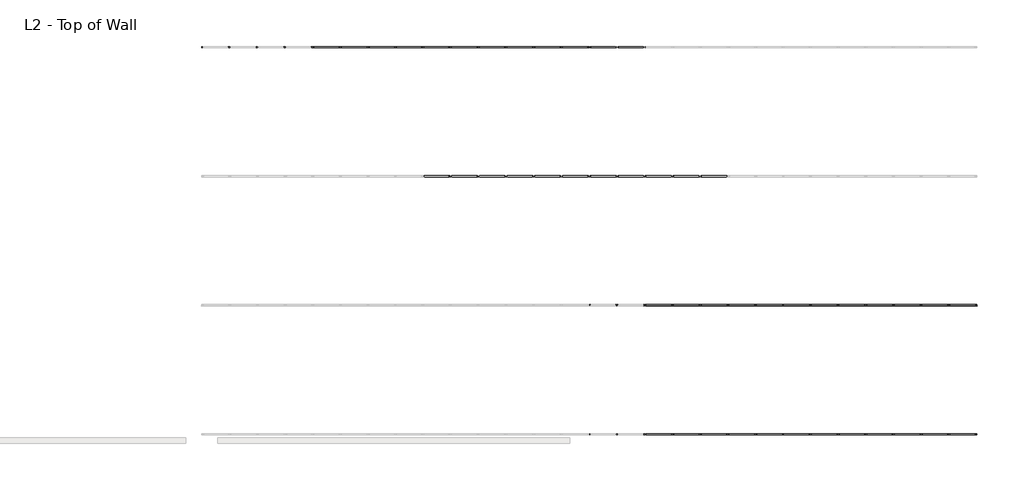
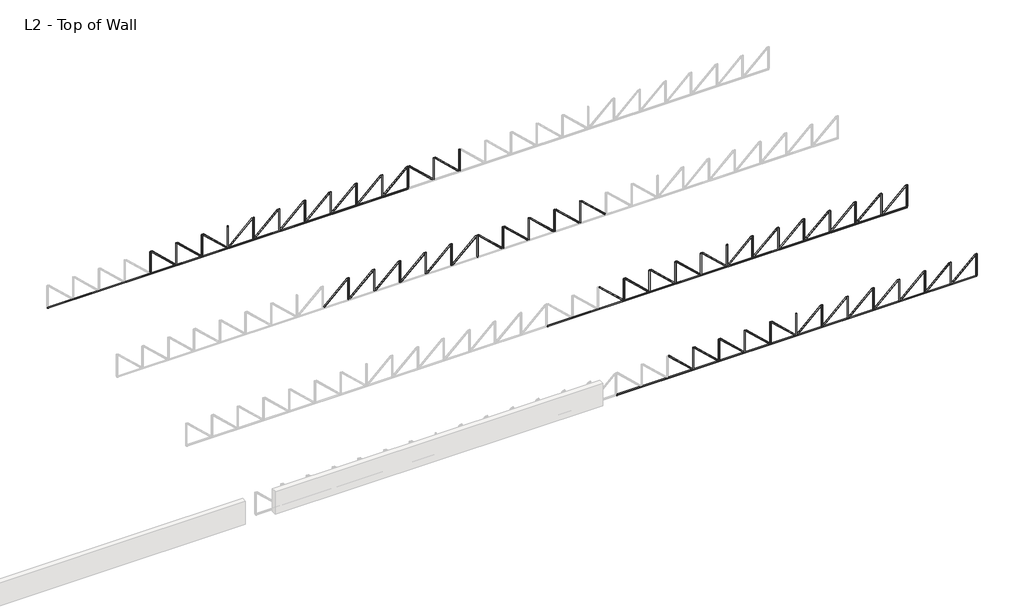
# One storey, part 2 of 4: 99 beams.
"""IFC4 building model written with IfcOpenShell, lengths in millimetres."""

import ifcopenshell
import ifcopenshell.guid

model = None  # the IFC model being written
_history = None  # IfcOwnerHistory: only IFC2X3 demands one
_inside = {}  # id of a spatial element -> (the spatial element, [elements in it])
_under = {}  # id of a project, library or spatial element -> (it, [spatial elements below it])
_declared = {}  # id of a project -> (the project, [libraries it declares])
_typed = {}  # id of a type object -> (the type object, [elements of that type])
_made_of = {}  # id of a material, layer set ... -> (it, [elements and type objects made of it])


def new_model(schema):
    """Start an empty IFC model of exactly this schema.

    Asked for "IFC4X3", IfcOpenShell would pick the latest addendum, in which some entities
    have other attributes; the version numbers below select the first issue.
    IFC2X3 requires an IfcOwnerHistory on every rooted entity: one is made here for all.
    """
    global model, _history
    if schema == "IFC4X3":
        model = ifcopenshell.file(schema_version=(4, 3, 0, 0))
    else:
        model = ifcopenshell.file(schema=schema)
    _inside.clear()
    _under.clear()
    _declared.clear()
    _typed.clear()
    _made_of.clear()
    _history = None
    if model.schema == "IFC2X3":
        org = make("IfcOrganization", Name="unknown")
        user = make(
            "IfcPersonAndOrganization",
            ThePerson=make("IfcPerson", FamilyName="unknown"),
            TheOrganization=org,
        )
        app = make(
            "IfcApplication",
            ApplicationDeveloper=org,
            Version="unknown",
            ApplicationFullName="unknown",
            ApplicationIdentifier="unknown",
        )
        _history = make(
            "IfcOwnerHistory",
            OwningUser=user,
            OwningApplication=app,
            ChangeAction="ADDED",
            CreationDate=0,
        )
    return model


def make(cls, **values):
    """One entity of the class cls with the attributes given. An attribute that is None is left unset."""
    return model.create_entity(
        cls, **{name: value for name, value in values.items() if value is not None}
    )


def rooted(cls, **values):
    """An entity with a GlobalId (a new one), such as an element, a storey or a relation."""
    return make(cls, GlobalId=ifcopenshell.guid.new(), OwnerHistory=_history, **values)


def si_unit(unit_type, name, prefix=None):
    """IfcSIUnit, for example si_unit("LENGTHUNIT", "METRE", prefix="MILLI")."""
    return make("IfcSIUnit", UnitType=unit_type, Prefix=prefix, Name=name)


def assignment(units):
    """IfcUnitAssignment: the units of a project."""
    return None if units is None else make("IfcUnitAssignment", Units=units)


def point(xyz):
    """IfcCartesianPoint."""
    return None if xyz is None else make("IfcCartesianPoint", Coordinates=xyz)


def direction(xyz):
    """IfcDirection."""
    return None if xyz is None else make("IfcDirection", DirectionRatios=xyz)


def frame(location, z_axis=None, x_axis=None):
    """IfcAxis2Placement3D, a coordinate frame: its origin and axes. An axis left out is left unset."""
    return make(
        "IfcAxis2Placement3D",
        Location=point(location),
        Axis=direction(z_axis),
        RefDirection=direction(x_axis),
    )


def frame_2d(location, x_axis=None):
    """IfcAxis2Placement2D, a coordinate frame in the plane: its origin and x axis."""
    return make(
        "IfcAxis2Placement2D", Location=point(location), RefDirection=direction(x_axis)
    )


def origin():
    """The frame at (0, 0, 0) with its axes left unset."""
    return frame((0.0, 0.0, 0.0))


def origin_2d():
    """The frame at (0, 0) in the plane with its x axis left unset."""
    return frame_2d((0.0, 0.0))


def place(relative_to, where):
    """IfcLocalPlacement: puts the frame where relative to a parent placement (None: the world)."""
    return make(
        "IfcLocalPlacement", PlacementRelTo=relative_to, RelativePlacement=where
    )


def context(
    kind, dimensions, precision=None, world=None, true_north=None, identifier=None
):
    """IfcGeometricRepresentationContext, for example the 3D "Model" context."""
    return make(
        "IfcGeometricRepresentationContext",
        ContextIdentifier=identifier,
        ContextType=kind,
        CoordinateSpaceDimension=dimensions,
        Precision=precision,
        WorldCoordinateSystem=world,
        TrueNorth=true_north,
    )


def project(units=None, contexts=None):
    """IfcProject with its units and contexts."""
    return rooted(
        "IfcProject",
        Name="project",
        RepresentationContexts=contexts,
        UnitsInContext=assignment(units),
    )


def spatial(cls, under=None, at=None, **own):
    """A site, building, storey or space (cls), placed at a placement, below another one or the project."""
    s = rooted(cls, ObjectPlacement=at, **own)
    if under is not None:
        _under.setdefault(under.id(), (under, []))[1].append(s)
    return s


def circle_curve(where, radius):
    """IfcCircle in the frame where."""
    return make("IfcCircle", Position=where, Radius=radius)


def trimmed(basis, trim1, trim2, sense, master):
    """IfcTrimmedCurve: the piece of a basis curve between two trims."""
    return make(
        "IfcTrimmedCurve",
        BasisCurve=basis,
        Trim1=trim1,
        Trim2=trim2,
        SenseAgreement=sense,
        MasterRepresentation=master,
    )


def segment(curve, same_sense, transition):
    """IfcCompositeCurveSegment."""
    return make(
        "IfcCompositeCurveSegment",
        Transition=transition,
        SameSense=same_sense,
        ParentCurve=curve,
    )


def composite_curve(segments, self_intersect=None):
    """IfcCompositeCurve: segments joined end to end."""
    return make("IfcCompositeCurve", Segments=segments, SelfIntersect=self_intersect)


def outline(outer, holes=None, kind="AREA"):
    """IfcArbitraryClosedProfileDef: a profile drawn as a closed curve; with holes, ...WithVoids."""
    if holes is None:
        return make("IfcArbitraryClosedProfileDef", ProfileType=kind, OuterCurve=outer)
    return make(
        "IfcArbitraryProfileDefWithVoids",
        ProfileType=kind,
        OuterCurve=outer,
        InnerCurves=holes,
    )


def extrude(swept, where, along, depth):
    """IfcExtrudedAreaSolid: the profile swept, set in the frame where, extruded along a direction by depth."""
    return make(
        "IfcExtrudedAreaSolid",
        SweptArea=swept,
        Position=where,
        ExtrudedDirection=direction(along),
        Depth=depth,
    )


def shape(context_of_items, identifier, shape_type, items):
    """IfcShapeRepresentation: the items that make up one representation, for example the "Body"."""
    return make(
        "IfcShapeRepresentation",
        ContextOfItems=context_of_items,
        RepresentationIdentifier=identifier,
        RepresentationType=shape_type,
        Items=items,
    )


def source(mapping_origin, context_of_items, identifier, shape_type, items):
    """IfcRepresentationMap: a shape defined once, which mapped items show again and again."""
    return make(
        "IfcRepresentationMap",
        MappingOrigin=mapping_origin,
        MappedRepresentation=shape(context_of_items, identifier, shape_type, items),
    )


def transform(
    local_origin,
    x_axis=None,
    y_axis=None,
    z_axis=None,
    scale=None,
    scale2=None,
    scale3=None,
    uniform=True,
):
    """IfcCartesianTransformationOperator3D, or its non-uniform kind. x_axis, y_axis, z_axis: its Axis1, 2, 3."""
    if uniform:
        return make(
            "IfcCartesianTransformationOperator3D",
            Axis1=direction(x_axis),
            Axis2=direction(y_axis),
            LocalOrigin=point(local_origin),
            Scale=scale,
            Axis3=direction(z_axis),
        )
    return make(
        "IfcCartesianTransformationOperator3DnonUniform",
        Axis1=direction(x_axis),
        Axis2=direction(y_axis),
        LocalOrigin=point(local_origin),
        Scale=scale,
        Axis3=direction(z_axis),
        Scale2=scale2,
        Scale3=scale3,
    )


def mapped(mapping_source, mapping_target):
    """IfcMappedItem: shows the shape of a source again, moved by a transform."""
    return make(
        "IfcMappedItem", MappingSource=mapping_source, MappingTarget=mapping_target
    )


def made_of(thing, what):
    """Note that an element or type object is made of a material, layer set ...; save() writes the relation."""
    if what is not None:
        _made_of.setdefault(what.id(), (what, []))[1].append(thing)
    return thing


def element(
    cls,
    number,
    at=None,
    inside=None,
    cuts=None,
    type_object=None,
    material=None,
    context=None,
    identifier="Body",
    shape_type=None,
    held_by="IfcProductDefinitionShape",
    body=None,
    shapes=None,
    **own,
):
    """One element of the class cls, such as IfcWall. Its Tag is "e" and its number.

    at: its placement. inside: the storey or other place that contains it. cuts: it is an
    opening in that element (IfcRelVoidsElement). A single representation is given by context,
    identifier, shape_type and body (its items); several are given by shapes. held_by: the class
    of the entity that holds the representations. save() writes the other relations.
    """
    e = rooted(cls, Tag="e%d" % number, ObjectPlacement=at, **own)
    if body is not None:
        shapes = [shape(context, identifier, shape_type, body)]
    if shapes is not None:
        e.Representation = make(held_by, Representations=shapes)
    if inside is not None:
        _inside.setdefault(inside.id(), (inside, []))[1].append(e)
    if cuts is not None:
        rooted(
            "IfcRelVoidsElement", RelatingBuildingElement=cuts, RelatedOpeningElement=e
        )
    if type_object is not None:
        _typed.setdefault(type_object.id(), (type_object, []))[1].append(e)
    return made_of(e, material)


def aggregate(whole, parts):
    """IfcRelAggregates: a whole, such as a stair, and the parts it consists of."""
    return rooted("IfcRelAggregates", RelatingObject=whole, RelatedObjects=parts)


def save(model, path):
    """Write the relations noted so far, then the file.

    IfcRelAggregates (storeys below a building ...), IfcRelContainedInSpatialStructure (elements
    in a storey), IfcRelDefinesByType, IfcRelAssociatesMaterial and IfcRelDeclares: one each for
    every whole, place, type object, material and project.
    """
    for whole, parts in _under.values():
        aggregate(whole, parts)
    for where, things in _inside.values():
        rooted(
            "IfcRelContainedInSpatialStructure",
            RelatedElements=things,
            RelatingStructure=where,
        )
    for kind, things in _typed.values():
        rooted("IfcRelDefinesByType", RelatedObjects=things, RelatingType=kind)
    for what, things in _made_of.values():
        rooted("IfcRelAssociatesMaterial", RelatedObjects=things, RelatingMaterial=what)
    for by, libraries in _declared.values():
        rooted("IfcRelDeclares", RelatingContext=by, RelatedDefinitions=libraries)
    model.write(path)


def circular_hollow_sections_chs60_3x5_c94bd862(model_context):
    return source(origin(), model_context, "Body", "SweptSolid", [
        extrude(outline(composite_curve([segment(trimmed(circle_curve(origin_2d(), 30.15), [point((-30.15, 0.0))], [point((30.15, 0.0))], False, "CARTESIAN"), True, "CONTINUOUS"), segment(trimmed(circle_curve(origin_2d(), 30.15), [point((30.15, 0.0))], [point((-30.15, 0.0))], False, "CARTESIAN"), True, "CONTINUOUS")], self_intersect=False), holes=[composite_curve([segment(trimmed(circle_curve(origin_2d(), 25.15), [point((25.15, 0.0))], [point((-25.15, 0.0))], True, "CARTESIAN"), True, "CONTINUOUS"), segment(trimmed(circle_curve(origin_2d(), 25.15), [point((-25.15, 0.0))], [point((25.15, 0.0))], True, "CARTESIAN"), True, "CONTINUOUS")], self_intersect=False)]), frame((-557.0, 0.0, 0.0), z_axis=(1.0, 0.0, 0.0), x_axis=(0.0, 1.0, 0.0)), (0.0, 0.0, 1.0), 1114.0),
    ])


def circular_hollow_sections_chs60_3x5_b8a643cb(model_context):
    return source(origin(), model_context, "Body", "SweptSolid", [
        extrude(outline(composite_curve([segment(trimmed(circle_curve(origin_2d(), 30.15), [point((-30.15, 0.0))], [point((30.15, 0.0))], False, "CARTESIAN"), True, "CONTINUOUS"), segment(trimmed(circle_curve(origin_2d(), 30.15), [point((30.15, 0.0))], [point((-30.15, 0.0))], False, "CARTESIAN"), True, "CONTINUOUS")], self_intersect=False), holes=[composite_curve([segment(trimmed(circle_curve(origin_2d(), 25.15), [point((25.15, 0.0))], [point((-25.15, 0.0))], True, "CARTESIAN"), True, "CONTINUOUS"), segment(trimmed(circle_curve(origin_2d(), 25.15), [point((-25.15, 0.0))], [point((25.15, 0.0))], True, "CARTESIAN"), True, "CONTINUOUS")], self_intersect=False)]), frame((-790.0, 0.0, 0.0), z_axis=(1.0, 0.0, 0.0), x_axis=(0.0, 1.0, 0.0)), (0.0, 0.0, 1.0), 1580.0),
    ])


def circular_hollow_sections_chs60_3x5_ee2473de(model_context):
    return source(origin(), model_context, "Body", "SweptSolid", [
        extrude(outline(composite_curve([segment(trimmed(circle_curve(origin_2d(), 30.15), [point((-30.15, 0.0))], [point((30.15, 0.0))], False, "CARTESIAN"), True, "CONTINUOUS"), segment(trimmed(circle_curve(origin_2d(), 30.15), [point((30.15, 0.0))], [point((-30.15, 0.0))], False, "CARTESIAN"), True, "CONTINUOUS")], self_intersect=False), holes=[composite_curve([segment(trimmed(circle_curve(origin_2d(), 25.15), [point((25.15, 0.0))], [point((-25.15, 0.0))], True, "CARTESIAN"), True, "CONTINUOUS"), segment(trimmed(circle_curve(origin_2d(), 25.15), [point((-25.15, 0.0))], [point((25.15, 0.0))], True, "CARTESIAN"), True, "CONTINUOUS")], self_intersect=False)]), frame((-9000.0, 0.0, 0.0), z_axis=(1.0, 0.0, 0.0), x_axis=(0.0, 1.0, 0.0)), (0.0, 0.0, 1.0), 18000.0),
    ])


def circular_hollow_sections_chs60_3x5_7809bf4e(model_context):
    return source(origin(), model_context, "Body", "SweptSolid", [
        extrude(outline(composite_curve([segment(trimmed(circle_curve(origin_2d(), 30.15), [point((-30.15, 0.0))], [point((30.15, 0.0))], False, "CARTESIAN"), True, "CONTINUOUS"), segment(trimmed(circle_curve(origin_2d(), 30.15), [point((30.15, 0.0))], [point((-30.15, 0.0))], False, "CARTESIAN"), True, "CONTINUOUS")], self_intersect=False), holes=[composite_curve([segment(trimmed(circle_curve(origin_2d(), 25.15), [point((25.15, 0.0))], [point((-25.15, 0.0))], True, "CARTESIAN"), True, "CONTINUOUS"), segment(trimmed(circle_curve(origin_2d(), 25.15), [point((-25.15, 0.0))], [point((25.15, 0.0))], True, "CARTESIAN"), True, "CONTINUOUS")], self_intersect=False)]), frame((-600.0, 0.0, 0.0), z_axis=(1.0, 0.0, 0.0), x_axis=(0.0, 1.0, 0.0)), (0.0, 0.0, 1.0), 1157.0),
    ])


model = new_model("IFC4")

# Units and contexts
model_context = context("Model", 3, world=origin())
ifc_project = project(units=[si_unit("LENGTHUNIT", "METRE", prefix="MILLI")], contexts=[model_context])

# Site, building, storey
site = spatial("IfcSite", under=ifc_project)
building = spatial("IfcBuilding", under=site)
storey = spatial("IfcBuildingStorey", under=building, Name="L2 - Top of Wall", Elevation=6600.0)

# Beams
placement = place(None, origin())
circular_hollow_sections_chs60_3x5_shape = circular_hollow_sections_chs60_3x5_c94bd862(model_context)
element("IfcBeam", 1, ObjectType="Circular Hollow Sections : CHS60.3x5", at=placement, inside=storey, context=model_context, shape_type="MappedRepresentation", body=[
    mapped(circular_hollow_sections_chs60_3x5_shape, transform((27576.1803686, -5058.7619082, 7200.0), x_axis=(0.0, 0.0, 1.0), y_axis=(0.0, -1.0, 0.0), z_axis=(1.0, 0.0, 0.0))),
])
element("IfcBeam", 2, ObjectType="Circular Hollow Sections : CHS60.3x5", at=placement, inside=storey, context=model_context, shape_type="MappedRepresentation", body=[
    mapped(circular_hollow_sections_chs60_3x5_shape, transform((26290.4660829, -5058.7619082, 7200.0), x_axis=(0.0, 0.0, 1.0), y_axis=(0.0, -1.0, 0.0), z_axis=(1.0, 0.0, 0.0))),
])
element("IfcBeam", 3, ObjectType="Circular Hollow Sections : CHS60.3x5", at=placement, inside=storey, context=model_context, shape_type="MappedRepresentation", body=[
    mapped(circular_hollow_sections_chs60_3x5_shape, transform((25004.7517972, -5058.7619082, 7200.0), x_axis=(0.0, 0.0, 1.0), y_axis=(0.0, -1.0, 0.0), z_axis=(1.0, 0.0, 0.0))),
])
element("IfcBeam", 4, ObjectType="Circular Hollow Sections : CHS60.3x5", at=placement, inside=storey, context=model_context, shape_type="MappedRepresentation", body=[
    mapped(circular_hollow_sections_chs60_3x5_shape, transform((23719.0375115, -5058.7619082, 7200.0), x_axis=(0.0, 0.0, 1.0), y_axis=(0.0, -1.0, 0.0), z_axis=(1.0, 0.0, 0.0))),
])
element("IfcBeam", 5, ObjectType="Circular Hollow Sections : CHS60.3x5", at=placement, inside=storey, context=model_context, shape_type="MappedRepresentation", body=[
    mapped(circular_hollow_sections_chs60_3x5_shape, transform((22433.3232257, -5058.7619082, 7200.0), x_axis=(0.0, 0.0, 1.0), y_axis=(0.0, -1.0, 0.0), z_axis=(1.0, 0.0, 0.0))),
])
element("IfcBeam", 6, ObjectType="Circular Hollow Sections : CHS60.3x5", at=placement, inside=storey, context=model_context, shape_type="MappedRepresentation", body=[
    mapped(circular_hollow_sections_chs60_3x5_shape, transform((28861.8946543, -5058.7619082, 7200.0), x_axis=(0.0, 0.0, 1.0), y_axis=(0.0, -1.0, 0.0), z_axis=(1.0, 0.0, 0.0))),
])
element("IfcBeam", 7, ObjectType="Circular Hollow Sections : CHS60.3x5", at=placement, inside=storey, context=model_context, shape_type="MappedRepresentation", body=[
    mapped(circular_hollow_sections_chs60_3x5_shape, transform((21147.60894, -5058.7619082, 7200.0), x_axis=(0.0, 0.0, 1.0), y_axis=(0.0, -1.0, 0.0), z_axis=(1.0, 0.0, 0.0))),
])
element("IfcBeam", 8, ObjectType="Circular Hollow Sections : CHS60.3x5", at=placement, inside=storey, context=model_context, shape_type="MappedRepresentation", body=[
    mapped(circular_hollow_sections_chs60_3x5_shape, transform((16004.7517972, -5058.7619082, 7200.0), x_axis=(0.0, 0.0, 1.0), y_axis=(0.0, -1.0, 0.0), z_axis=(1.0, 0.0, 0.0))),
])
element("IfcBeam", 9, ObjectType="Circular Hollow Sections : CHS60.3x5", at=placement, inside=storey, context=model_context, shape_type="MappedRepresentation", body=[
    mapped(circular_hollow_sections_chs60_3x5_shape, transform((17290.4660829, -5058.7619082, 7200.0), x_axis=(0.0, 0.0, 1.0), y_axis=(0.0, -1.0, 0.0), z_axis=(1.0, 0.0, 0.0))),
])
element("IfcBeam", 10, ObjectType="Circular Hollow Sections : CHS60.3x5", at=placement, inside=storey, context=model_context, shape_type="MappedRepresentation", body=[
    mapped(circular_hollow_sections_chs60_3x5_shape, transform((18576.1803686, -5058.7619082, 7200.0), x_axis=(0.0, 0.0, 1.0), y_axis=(0.0, -1.0, 0.0), z_axis=(1.0, 0.0, 0.0))),
])
element("IfcBeam", 11, ObjectType="Circular Hollow Sections : CHS60.3x5", at=placement, inside=storey, context=model_context, shape_type="MappedRepresentation", body=[
    mapped(circular_hollow_sections_chs60_3x5_shape, transform((19861.8946543, -5058.7619082, 7200.0), x_axis=(0.0, 0.0, 1.0), y_axis=(0.0, -1.0, 0.0), z_axis=(1.0, 0.0, 0.0))),
])
element("IfcBeam", 12, ObjectType="Circular Hollow Sections : CHS60.3x5", at=placement, inside=storey, context=model_context, shape_type="MappedRepresentation", body=[
    mapped(circular_hollow_sections_chs60_3x5_shape, transform((27574.7303686, -11058.7619082, 7200.0), x_axis=(0.0, 0.0, 1.0), y_axis=(0.0, -1.0, 0.0), z_axis=(1.0, 0.0, 0.0))),
])
element("IfcBeam", 13, ObjectType="Circular Hollow Sections : CHS60.3x5", at=placement, inside=storey, context=model_context, shape_type="MappedRepresentation", body=[
    mapped(circular_hollow_sections_chs60_3x5_shape, transform((26289.0160829, -11058.7619082, 7200.0), x_axis=(0.0, 0.0, 1.0), y_axis=(0.0, -1.0, 0.0), z_axis=(1.0, 0.0, 0.0))),
])
element("IfcBeam", 14, ObjectType="Circular Hollow Sections : CHS60.3x5", at=placement, inside=storey, context=model_context, shape_type="MappedRepresentation", body=[
    mapped(circular_hollow_sections_chs60_3x5_shape, transform((25003.3017972, -11058.7619082, 7200.0), x_axis=(0.0, 0.0, 1.0), y_axis=(0.0, -1.0, 0.0), z_axis=(1.0, 0.0, 0.0))),
])
element("IfcBeam", 15, ObjectType="Circular Hollow Sections : CHS60.3x5", at=placement, inside=storey, context=model_context, shape_type="MappedRepresentation", body=[
    mapped(circular_hollow_sections_chs60_3x5_shape, transform((23717.5875115, -11058.7619082, 7200.0), x_axis=(0.0, 0.0, 1.0), y_axis=(0.0, -1.0, 0.0), z_axis=(1.0, 0.0, 0.0))),
])
element("IfcBeam", 16, ObjectType="Circular Hollow Sections : CHS60.3x5", at=placement, inside=storey, context=model_context, shape_type="MappedRepresentation", body=[
    mapped(circular_hollow_sections_chs60_3x5_shape, transform((22431.8732257, -11058.7619082, 7200.0), x_axis=(0.0, 0.0, 1.0), y_axis=(0.0, -1.0, 0.0), z_axis=(1.0, 0.0, 0.0))),
])
element("IfcBeam", 17, ObjectType="Circular Hollow Sections : CHS60.3x5", at=placement, inside=storey, context=model_context, shape_type="MappedRepresentation", body=[
    mapped(circular_hollow_sections_chs60_3x5_shape, transform((28860.4446543, -11058.7619082, 7200.0), x_axis=(0.0, 0.0, 1.0), y_axis=(0.0, -1.0, 0.0), z_axis=(1.0, 0.0, 0.0))),
])
element("IfcBeam", 18, ObjectType="Circular Hollow Sections : CHS60.3x5", at=placement, inside=storey, context=model_context, shape_type="MappedRepresentation", body=[
    mapped(circular_hollow_sections_chs60_3x5_shape, transform((45574.7303686, -17058.7619082, 7200.0), x_axis=(0.0, 0.0, 1.0), y_axis=(0.0, -1.0, 0.0), z_axis=(1.0, 0.0, 0.0))),
])
element("IfcBeam", 19, ObjectType="Circular Hollow Sections : CHS60.3x5", at=placement, inside=storey, context=model_context, shape_type="MappedRepresentation", body=[
    mapped(circular_hollow_sections_chs60_3x5_shape, transform((44289.0160829, -17058.7619082, 7200.0), x_axis=(0.0, 0.0, 1.0), y_axis=(0.0, -1.0, 0.0), z_axis=(1.0, 0.0, 0.0))),
])
element("IfcBeam", 20, ObjectType="Circular Hollow Sections : CHS60.3x5", at=placement, inside=storey, context=model_context, shape_type="MappedRepresentation", body=[
    mapped(circular_hollow_sections_chs60_3x5_shape, transform((43003.3017972, -17058.7619082, 7200.0), x_axis=(0.0, 0.0, 1.0), y_axis=(0.0, -1.0, 0.0), z_axis=(1.0, 0.0, 0.0))),
])
element("IfcBeam", 21, ObjectType="Circular Hollow Sections : CHS60.3x5", at=placement, inside=storey, context=model_context, shape_type="MappedRepresentation", body=[
    mapped(circular_hollow_sections_chs60_3x5_shape, transform((32717.5875115, -17058.7619082, 7200.0), x_axis=(0.0, 0.0, 1.0), y_axis=(0.0, -1.0, 0.0), z_axis=(1.0, 0.0, 0.0))),
])
element("IfcBeam", 22, ObjectType="Circular Hollow Sections : CHS60.3x5", at=placement, inside=storey, context=model_context, shape_type="MappedRepresentation", body=[
    mapped(circular_hollow_sections_chs60_3x5_shape, transform((41717.5875115, -17058.7619082, 7200.0), x_axis=(0.0, 0.0, 1.0), y_axis=(0.0, -1.0, 0.0), z_axis=(1.0, 0.0, 0.0))),
])
element("IfcBeam", 23, ObjectType="Circular Hollow Sections : CHS60.3x5", at=placement, inside=storey, context=model_context, shape_type="MappedRepresentation", body=[
    mapped(circular_hollow_sections_chs60_3x5_shape, transform((40431.8732257, -17058.7619082, 7200.0), x_axis=(0.0, 0.0, 1.0), y_axis=(0.0, -1.0, 0.0), z_axis=(1.0, 0.0, 0.0))),
])
element("IfcBeam", 24, ObjectType="Circular Hollow Sections : CHS60.3x5", at=placement, inside=storey, context=model_context, shape_type="MappedRepresentation", body=[
    mapped(circular_hollow_sections_chs60_3x5_shape, transform((46860.4446543, -17058.7619082, 7200.0), x_axis=(0.0, 0.0, 1.0), y_axis=(0.0, -1.0, 0.0), z_axis=(1.0, 0.0, 0.0))),
])
element("IfcBeam", 25, ObjectType="Circular Hollow Sections : CHS60.3x5", at=placement, inside=storey, context=model_context, shape_type="MappedRepresentation", body=[
    mapped(circular_hollow_sections_chs60_3x5_shape, transform((39146.15894, -17058.7619082, 7200.0), x_axis=(0.0, 0.0, 1.0), y_axis=(0.0, -1.0, 0.0), z_axis=(1.0, 0.0, 0.0))),
])
element("IfcBeam", 26, ObjectType="Circular Hollow Sections : CHS60.3x5", at=placement, inside=storey, context=model_context, shape_type="MappedRepresentation", body=[
    mapped(circular_hollow_sections_chs60_3x5_shape, transform((34003.3017972, -17058.7619082, 7200.0), x_axis=(0.0, 0.0, 1.0), y_axis=(0.0, -1.0, 0.0), z_axis=(1.0, 0.0, 0.0))),
])
element("IfcBeam", 27, ObjectType="Circular Hollow Sections : CHS60.3x5", at=placement, inside=storey, context=model_context, shape_type="MappedRepresentation", body=[
    mapped(circular_hollow_sections_chs60_3x5_shape, transform((35289.0160829, -17058.7619082, 7200.0), x_axis=(0.0, 0.0, 1.0), y_axis=(0.0, -1.0, 0.0), z_axis=(1.0, 0.0, 0.0))),
])
element("IfcBeam", 28, ObjectType="Circular Hollow Sections : CHS60.3x5", at=placement, inside=storey, context=model_context, shape_type="MappedRepresentation", body=[
    mapped(circular_hollow_sections_chs60_3x5_shape, transform((36574.7303686, -17058.7619082, 7200.0), x_axis=(0.0, 0.0, 1.0), y_axis=(0.0, -1.0, 0.0), z_axis=(1.0, 0.0, 0.0))),
])
element("IfcBeam", 29, ObjectType="Circular Hollow Sections : CHS60.3x5", at=placement, inside=storey, context=model_context, shape_type="MappedRepresentation", body=[
    mapped(circular_hollow_sections_chs60_3x5_shape, transform((37860.4446543, -17058.7619082, 7200.0), x_axis=(0.0, 0.0, 1.0), y_axis=(0.0, -1.0, 0.0), z_axis=(1.0, 0.0, 0.0))),
])
element("IfcBeam", 30, ObjectType="Circular Hollow Sections : CHS60.3x5", at=placement, inside=storey, context=model_context, shape_type="MappedRepresentation", body=[
    mapped(circular_hollow_sections_chs60_3x5_shape, transform((45574.7303686, -23058.7619082, 7200.0), x_axis=(0.0, 0.0, 1.0), y_axis=(0.0, -1.0, 0.0), z_axis=(1.0, 0.0, 0.0))),
])
element("IfcBeam", 31, ObjectType="Circular Hollow Sections : CHS60.3x5", at=placement, inside=storey, context=model_context, shape_type="MappedRepresentation", body=[
    mapped(circular_hollow_sections_chs60_3x5_shape, transform((44289.0160829, -23058.7619082, 7200.0), x_axis=(0.0, 0.0, 1.0), y_axis=(0.0, -1.0, 0.0), z_axis=(1.0, 0.0, 0.0))),
])
element("IfcBeam", 32, ObjectType="Circular Hollow Sections : CHS60.3x5", at=placement, inside=storey, context=model_context, shape_type="MappedRepresentation", body=[
    mapped(circular_hollow_sections_chs60_3x5_shape, transform((43003.3017972, -23058.7619082, 7200.0), x_axis=(0.0, 0.0, 1.0), y_axis=(0.0, -1.0, 0.0), z_axis=(1.0, 0.0, 0.0))),
])
element("IfcBeam", 33, ObjectType="Circular Hollow Sections : CHS60.3x5", at=placement, inside=storey, context=model_context, shape_type="MappedRepresentation", body=[
    mapped(circular_hollow_sections_chs60_3x5_shape, transform((32717.5875115, -23058.7619082, 7200.0), x_axis=(0.0, 0.0, 1.0), y_axis=(0.0, -1.0, 0.0), z_axis=(1.0, 0.0, 0.0))),
])
element("IfcBeam", 34, ObjectType="Circular Hollow Sections : CHS60.3x5", at=placement, inside=storey, context=model_context, shape_type="MappedRepresentation", body=[
    mapped(circular_hollow_sections_chs60_3x5_shape, transform((41717.5875115, -23058.7619082, 7200.0), x_axis=(0.0, 0.0, 1.0), y_axis=(0.0, -1.0, 0.0), z_axis=(1.0, 0.0, 0.0))),
])
element("IfcBeam", 35, ObjectType="Circular Hollow Sections : CHS60.3x5", at=placement, inside=storey, context=model_context, shape_type="MappedRepresentation", body=[
    mapped(circular_hollow_sections_chs60_3x5_shape, transform((40431.8732257, -23058.7619082, 7200.0), x_axis=(0.0, 0.0, 1.0), y_axis=(0.0, -1.0, 0.0), z_axis=(1.0, 0.0, 0.0))),
])
element("IfcBeam", 36, ObjectType="Circular Hollow Sections : CHS60.3x5", at=placement, inside=storey, context=model_context, shape_type="MappedRepresentation", body=[
    mapped(circular_hollow_sections_chs60_3x5_shape, transform((46860.4446543, -23058.7619082, 7200.0), x_axis=(0.0, 0.0, 1.0), y_axis=(0.0, -1.0, 0.0), z_axis=(1.0, 0.0, 0.0))),
])
element("IfcBeam", 37, ObjectType="Circular Hollow Sections : CHS60.3x5", at=placement, inside=storey, context=model_context, shape_type="MappedRepresentation", body=[
    mapped(circular_hollow_sections_chs60_3x5_shape, transform((39146.15894, -23058.7619082, 7200.0), x_axis=(0.0, 0.0, 1.0), y_axis=(0.0, -1.0, 0.0), z_axis=(1.0, 0.0, 0.0))),
])
element("IfcBeam", 38, ObjectType="Circular Hollow Sections : CHS60.3x5", at=placement, inside=storey, context=model_context, shape_type="MappedRepresentation", body=[
    mapped(circular_hollow_sections_chs60_3x5_shape, transform((34003.3017972, -23058.7619082, 7200.0), x_axis=(0.0, 0.0, 1.0), y_axis=(0.0, -1.0, 0.0), z_axis=(1.0, 0.0, 0.0))),
])
element("IfcBeam", 39, ObjectType="Circular Hollow Sections : CHS60.3x5", at=placement, inside=storey, context=model_context, shape_type="MappedRepresentation", body=[
    mapped(circular_hollow_sections_chs60_3x5_shape, transform((35289.0160829, -23058.7619082, 7200.0), x_axis=(0.0, 0.0, 1.0), y_axis=(0.0, -1.0, 0.0), z_axis=(1.0, 0.0, 0.0))),
])
element("IfcBeam", 40, ObjectType="Circular Hollow Sections : CHS60.3x5", at=placement, inside=storey, context=model_context, shape_type="MappedRepresentation", body=[
    mapped(circular_hollow_sections_chs60_3x5_shape, transform((36574.7303686, -23058.7619082, 7200.0), x_axis=(0.0, 0.0, 1.0), y_axis=(0.0, -1.0, 0.0), z_axis=(1.0, 0.0, 0.0))),
])
element("IfcBeam", 41, ObjectType="Circular Hollow Sections : CHS60.3x5", at=placement, inside=storey, context=model_context, shape_type="MappedRepresentation", body=[
    mapped(circular_hollow_sections_chs60_3x5_shape, transform((37860.4446543, -23058.7619082, 7200.0), x_axis=(0.0, 0.0, 1.0), y_axis=(0.0, -1.0, 0.0), z_axis=(1.0, 0.0, 0.0))),
])
element("IfcBeam", 42, ObjectType="Circular Hollow Sections : CHS60.3x5", at=placement, inside=storey, context=model_context, shape_type="MappedRepresentation", body=[
    mapped(circular_hollow_sections_chs60_3x5_shape, transform((30147.60894, -5058.7619082, 7200.0), x_axis=(0.0, 0.0, 1.0000000000000002), y_axis=(0.0, -1.0000000000000002, 0.0), z_axis=(1.0000000000000002, 0.0, 0.0))),
])
element("IfcBeam", 43, ObjectType="Circular Hollow Sections : CHS60.3x5", at=placement, inside=storey, context=model_context, shape_type="MappedRepresentation", body=[
    mapped(circular_hollow_sections_chs60_3x5_shape, transform((31433.3232257, -5058.7619082, 7200.0), x_axis=(0.0, 0.0, 1.0000000000000002), y_axis=(0.0, -1.0000000000000002, 0.0), z_axis=(1.0000000000000002, 0.0, 0.0))),
])
element("IfcBeam", 44, ObjectType="Circular Hollow Sections : CHS60.3x5", at=placement, inside=storey, context=model_context, shape_type="MappedRepresentation", body=[
    mapped(circular_hollow_sections_chs60_3x5_shape, transform((30147.60894, -11058.7619082, 7200.0), x_axis=(0.0, 0.0, 1.0000000000000002), y_axis=(0.0, -1.0000000000000002, 0.0), z_axis=(1.0000000000000002, 0.0, 0.0))),
])
element("IfcBeam", 45, ObjectType="Circular Hollow Sections : CHS60.3x5", at=placement, inside=storey, context=model_context, shape_type="MappedRepresentation", body=[
    mapped(circular_hollow_sections_chs60_3x5_shape, transform((31433.3232257, -11058.7619082, 7200.0), x_axis=(0.0, 0.0, 1.0000000000000002), y_axis=(0.0, -1.0000000000000002, 0.0), z_axis=(1.0000000000000002, 0.0, 0.0))),
])
element("IfcBeam", 46, ObjectType="Circular Hollow Sections : CHS60.3x5", at=placement, inside=storey, context=model_context, shape_type="MappedRepresentation", body=[
    mapped(circular_hollow_sections_chs60_3x5_shape, transform((32719.0375115, -11058.7619082, 7200.0), x_axis=(0.0, 0.0, 1.0000000000000002), y_axis=(0.0, -1.0000000000000002, 0.0), z_axis=(1.0000000000000002, 0.0, 0.0))),
])
element("IfcBeam", 47, ObjectType="Circular Hollow Sections : CHS60.3x5", at=placement, inside=storey, context=model_context, shape_type="MappedRepresentation", body=[
    mapped(circular_hollow_sections_chs60_3x5_shape, transform((34004.7517972, -11058.7619082, 7200.0), x_axis=(0.0, 0.0, 1.0000000000000002), y_axis=(0.0, -1.0000000000000002, 0.0), z_axis=(1.0000000000000002, 0.0, 0.0))),
])
circular_hollow_sections_chs60_3x5_2_shape = circular_hollow_sections_chs60_3x5_b8a643cb(model_context)
element("IfcBeam", 48, ObjectType="Circular Hollow Sections : CHS60.3x5", at=placement, inside=storey, context=model_context, shape_type="MappedRepresentation", body=[
    mapped(circular_hollow_sections_chs60_3x5_2_shape, transform((26933.3232257, -5058.7619082, 7200.0), x_axis=(0.7310552682428697, 0.0, 0.6823182503600105), y_axis=(0.0, -1.0, 0.0), z_axis=(0.6823182503600105, 0.0, -0.7310552682428697))),
])
element("IfcBeam", 49, ObjectType="Circular Hollow Sections : CHS60.3x5", at=placement, inside=storey, context=model_context, shape_type="MappedRepresentation", body=[
    mapped(circular_hollow_sections_chs60_3x5_2_shape, transform((25647.60894, -5058.7619082, 7200.0), x_axis=(0.7310552682428697, 0.0, 0.6823182503600105), y_axis=(0.0, -1.0, 0.0), z_axis=(0.6823182503600105, 0.0, -0.7310552682428697))),
])
element("IfcBeam", 50, ObjectType="Circular Hollow Sections : CHS60.3x5", at=placement, inside=storey, context=model_context, shape_type="MappedRepresentation", body=[
    mapped(circular_hollow_sections_chs60_3x5_2_shape, transform((24361.8946543, -5058.7619082, 7200.0), x_axis=(0.7310552682428697, 0.0, 0.6823182503600105), y_axis=(0.0, -1.0, 0.0), z_axis=(0.6823182503600105, 0.0, -0.7310552682428697))),
])
element("IfcBeam", 51, ObjectType="Circular Hollow Sections : CHS60.3x5", at=placement, inside=storey, context=model_context, shape_type="MappedRepresentation", body=[
    mapped(circular_hollow_sections_chs60_3x5_2_shape, transform((23076.1803686, -5058.7619082, 7200.0), x_axis=(0.7310552682428697, 0.0, 0.6823182503600105), y_axis=(0.0, -1.0, 0.0), z_axis=(0.6823182503600105, 0.0, -0.7310552682428697))),
])
element("IfcBeam", 52, ObjectType="Circular Hollow Sections : CHS60.3x5", at=placement, inside=storey, context=model_context, shape_type="MappedRepresentation", body=[
    mapped(circular_hollow_sections_chs60_3x5_2_shape, transform((21790.4660829, -5058.7619082, 7200.0), x_axis=(0.7310552682428697, 0.0, 0.6823182503600105), y_axis=(0.0, -1.0, 0.0), z_axis=(0.6823182503600105, 0.0, -0.7310552682428697))),
])
element("IfcBeam", 53, ObjectType="Circular Hollow Sections : CHS60.3x5", at=placement, inside=storey, context=model_context, shape_type="MappedRepresentation", body=[
    mapped(circular_hollow_sections_chs60_3x5_2_shape, transform((28219.0375115, -5058.7619082, 7200.0), x_axis=(0.7310552682428697, 0.0, 0.6823182503600105), y_axis=(0.0, -1.0, 0.0), z_axis=(0.6823182503600105, 0.0, -0.7310552682428697))),
])
element("IfcBeam", 54, ObjectType="Circular Hollow Sections : CHS60.3x5", at=placement, inside=storey, context=model_context, shape_type="MappedRepresentation", body=[
    mapped(circular_hollow_sections_chs60_3x5_2_shape, transform((20504.7517972, -5058.7619082, 7200.0), x_axis=(0.7310552682428697, 0.0, 0.6823182503600105), y_axis=(0.0, -1.0, 0.0), z_axis=(0.6823182503600105, 0.0, -0.7310552682428697))),
])
element("IfcBeam", 55, ObjectType="Circular Hollow Sections : CHS60.3x5", at=placement, inside=storey, context=model_context, shape_type="MappedRepresentation", body=[
    mapped(circular_hollow_sections_chs60_3x5_2_shape, transform((16647.60894, -5058.7619082, 7200.0), x_axis=(0.7310552682428691, 0.0, -0.6823182503600111), y_axis=(0.0, -1.0, 0.0), z_axis=(-0.6823182503600111, 0.0, -0.7310552682428691))),
])
element("IfcBeam", 56, ObjectType="Circular Hollow Sections : CHS60.3x5", at=placement, inside=storey, context=model_context, shape_type="MappedRepresentation", body=[
    mapped(circular_hollow_sections_chs60_3x5_2_shape, transform((17933.3232257, -5058.7619082, 7200.0), x_axis=(0.7310552682428691, 0.0, -0.6823182503600111), y_axis=(0.0, -1.0, 0.0), z_axis=(-0.6823182503600111, 0.0, -0.7310552682428691))),
])
element("IfcBeam", 57, ObjectType="Circular Hollow Sections : CHS60.3x5", at=placement, inside=storey, context=model_context, shape_type="MappedRepresentation", body=[
    mapped(circular_hollow_sections_chs60_3x5_2_shape, transform((19219.0375115, -5058.7619082, 7200.0), x_axis=(0.7310552682428686, 0.0, -0.6823182503600118), y_axis=(0.0, -1.0, 0.0), z_axis=(-0.6823182503600118, 0.0, -0.7310552682428686))),
])
element("IfcBeam", 58, ObjectType="Circular Hollow Sections : CHS60.3x5", at=placement, inside=storey, context=model_context, shape_type="MappedRepresentation", body=[
    mapped(circular_hollow_sections_chs60_3x5_2_shape, transform((26931.8732257, -11058.7619082, 7200.0), x_axis=(0.7310552682428697, 0.0, 0.6823182503600105), y_axis=(0.0, -1.0, 0.0), z_axis=(0.6823182503600105, 0.0, -0.7310552682428697))),
])
element("IfcBeam", 59, ObjectType="Circular Hollow Sections : CHS60.3x5", at=placement, inside=storey, context=model_context, shape_type="MappedRepresentation", body=[
    mapped(circular_hollow_sections_chs60_3x5_2_shape, transform((25646.15894, -11058.7619082, 7200.0), x_axis=(0.7310552682428697, 0.0, 0.6823182503600105), y_axis=(0.0, -1.0, 0.0), z_axis=(0.6823182503600105, 0.0, -0.7310552682428697))),
])
element("IfcBeam", 60, ObjectType="Circular Hollow Sections : CHS60.3x5", at=placement, inside=storey, context=model_context, shape_type="MappedRepresentation", body=[
    mapped(circular_hollow_sections_chs60_3x5_2_shape, transform((24360.4446543, -11058.7619082, 7200.0), x_axis=(0.7310552682428697, 0.0, 0.6823182503600105), y_axis=(0.0, -1.0, 0.0), z_axis=(0.6823182503600105, 0.0, -0.7310552682428697))),
])
element("IfcBeam", 61, ObjectType="Circular Hollow Sections : CHS60.3x5", at=placement, inside=storey, context=model_context, shape_type="MappedRepresentation", body=[
    mapped(circular_hollow_sections_chs60_3x5_2_shape, transform((23074.7303686, -11058.7619082, 7200.0), x_axis=(0.7310552682428697, 0.0, 0.6823182503600105), y_axis=(0.0, -1.0, 0.0), z_axis=(0.6823182503600105, 0.0, -0.7310552682428697))),
])
element("IfcBeam", 62, ObjectType="Circular Hollow Sections : CHS60.3x5", at=placement, inside=storey, context=model_context, shape_type="MappedRepresentation", body=[
    mapped(circular_hollow_sections_chs60_3x5_2_shape, transform((21789.0160829, -11058.7619082, 7200.0), x_axis=(0.7310552682428697, 0.0, 0.6823182503600105), y_axis=(0.0, -1.0, 0.0), z_axis=(0.6823182503600105, 0.0, -0.7310552682428697))),
])
element("IfcBeam", 63, ObjectType="Circular Hollow Sections : CHS60.3x5", at=placement, inside=storey, context=model_context, shape_type="MappedRepresentation", body=[
    mapped(circular_hollow_sections_chs60_3x5_2_shape, transform((28217.5875115, -11058.7619082, 7200.0), x_axis=(0.7310552682428697, 0.0, 0.6823182503600105), y_axis=(0.0, -1.0, 0.0), z_axis=(0.6823182503600105, 0.0, -0.7310552682428697))),
])
element("IfcBeam", 64, ObjectType="Circular Hollow Sections : CHS60.3x5", at=placement, inside=storey, context=model_context, shape_type="MappedRepresentation", body=[
    mapped(circular_hollow_sections_chs60_3x5_2_shape, transform((44931.8732257, -17058.7619082, 7200.0), x_axis=(0.7310552682428697, 0.0, 0.6823182503600105), y_axis=(0.0, -1.0, 0.0), z_axis=(0.6823182503600105, 0.0, -0.7310552682428697))),
])
element("IfcBeam", 65, ObjectType="Circular Hollow Sections : CHS60.3x5", at=placement, inside=storey, context=model_context, shape_type="MappedRepresentation", body=[
    mapped(circular_hollow_sections_chs60_3x5_2_shape, transform((43646.15894, -17058.7619082, 7200.0), x_axis=(0.7310552682428697, 0.0, 0.6823182503600105), y_axis=(0.0, -1.0, 0.0), z_axis=(0.6823182503600105, 0.0, -0.7310552682428697))),
])
element("IfcBeam", 66, ObjectType="Circular Hollow Sections : CHS60.3x5", at=placement, inside=storey, context=model_context, shape_type="MappedRepresentation", body=[
    mapped(circular_hollow_sections_chs60_3x5_2_shape, transform((32074.7303686, -17058.7619082, 7200.0), x_axis=(0.7310552682428686, 0.0, -0.6823182503600118), y_axis=(0.0, -1.0, 0.0), z_axis=(-0.6823182503600118, 0.0, -0.7310552682428686))),
])
element("IfcBeam", 67, ObjectType="Circular Hollow Sections : CHS60.3x5", at=placement, inside=storey, context=model_context, shape_type="MappedRepresentation", body=[
    mapped(circular_hollow_sections_chs60_3x5_2_shape, transform((42360.4446543, -17058.7619082, 7200.0), x_axis=(0.7310552682428697, 0.0, 0.6823182503600105), y_axis=(0.0, -1.0, 0.0), z_axis=(0.6823182503600105, 0.0, -0.7310552682428697))),
])
element("IfcBeam", 68, ObjectType="Circular Hollow Sections : CHS60.3x5", at=placement, inside=storey, context=model_context, shape_type="MappedRepresentation", body=[
    mapped(circular_hollow_sections_chs60_3x5_2_shape, transform((33360.4446543, -17058.7619082, 7200.0), x_axis=(0.7310552682428686, 0.0, -0.6823182503600118), y_axis=(0.0, -1.0, 0.0), z_axis=(-0.6823182503600118, 0.0, -0.7310552682428686))),
])
element("IfcBeam", 69, ObjectType="Circular Hollow Sections : CHS60.3x5", at=placement, inside=storey, context=model_context, shape_type="MappedRepresentation", body=[
    mapped(circular_hollow_sections_chs60_3x5_2_shape, transform((41074.7303686, -17058.7619082, 7200.0), x_axis=(0.7310552682428697, 0.0, 0.6823182503600105), y_axis=(0.0, -1.0, 0.0), z_axis=(0.6823182503600105, 0.0, -0.7310552682428697))),
])
element("IfcBeam", 70, ObjectType="Circular Hollow Sections : CHS60.3x5", at=placement, inside=storey, context=model_context, shape_type="MappedRepresentation", body=[
    mapped(circular_hollow_sections_chs60_3x5_2_shape, transform((39789.0160829, -17058.7619082, 7200.0), x_axis=(0.7310552682428697, 0.0, 0.6823182503600105), y_axis=(0.0, -1.0, 0.0), z_axis=(0.6823182503600105, 0.0, -0.7310552682428697))),
])
element("IfcBeam", 71, ObjectType="Circular Hollow Sections : CHS60.3x5", at=placement, inside=storey, context=model_context, shape_type="MappedRepresentation", body=[
    mapped(circular_hollow_sections_chs60_3x5_2_shape, transform((46217.5875115, -17058.7619082, 7200.0), x_axis=(0.7310552682428697, 0.0, 0.6823182503600105), y_axis=(0.0, -1.0, 0.0), z_axis=(0.6823182503600105, 0.0, -0.7310552682428697))),
])
element("IfcBeam", 72, ObjectType="Circular Hollow Sections : CHS60.3x5", at=placement, inside=storey, context=model_context, shape_type="MappedRepresentation", body=[
    mapped(circular_hollow_sections_chs60_3x5_2_shape, transform((38503.3017972, -17058.7619082, 7200.0), x_axis=(0.7310552682428697, 0.0, 0.6823182503600105), y_axis=(0.0, -1.0, 0.0), z_axis=(0.6823182503600105, 0.0, -0.7310552682428697))),
])
element("IfcBeam", 73, ObjectType="Circular Hollow Sections : CHS60.3x5", at=placement, inside=storey, context=model_context, shape_type="MappedRepresentation", body=[
    mapped(circular_hollow_sections_chs60_3x5_2_shape, transform((34646.15894, -17058.7619082, 7200.0), x_axis=(0.7310552682428686, 0.0, -0.6823182503600118), y_axis=(0.0, -1.0, 0.0), z_axis=(-0.6823182503600118, 0.0, -0.7310552682428686))),
])
element("IfcBeam", 74, ObjectType="Circular Hollow Sections : CHS60.3x5", at=placement, inside=storey, context=model_context, shape_type="MappedRepresentation", body=[
    mapped(circular_hollow_sections_chs60_3x5_2_shape, transform((35931.8732257, -17058.7619082, 7200.0), x_axis=(0.7310552682428686, 0.0, -0.6823182503600118), y_axis=(0.0, -1.0, 0.0), z_axis=(-0.6823182503600118, 0.0, -0.7310552682428686))),
])
element("IfcBeam", 75, ObjectType="Circular Hollow Sections : CHS60.3x5", at=placement, inside=storey, context=model_context, shape_type="MappedRepresentation", body=[
    mapped(circular_hollow_sections_chs60_3x5_2_shape, transform((37217.5875115, -17058.7619082, 7200.0), x_axis=(0.7310552682428686, 0.0, -0.6823182503600118), y_axis=(0.0, -1.0, 0.0), z_axis=(-0.6823182503600118, 0.0, -0.7310552682428686))),
])
element("IfcBeam", 76, ObjectType="Circular Hollow Sections : CHS60.3x5", at=placement, inside=storey, context=model_context, shape_type="MappedRepresentation", body=[
    mapped(circular_hollow_sections_chs60_3x5_2_shape, transform((44931.8732257, -23058.7619082, 7200.0), x_axis=(0.7310552682428697, 0.0, 0.6823182503600105), y_axis=(0.0, -1.0, 0.0), z_axis=(0.6823182503600105, 0.0, -0.7310552682428697))),
])
element("IfcBeam", 77, ObjectType="Circular Hollow Sections : CHS60.3x5", at=placement, inside=storey, context=model_context, shape_type="MappedRepresentation", body=[
    mapped(circular_hollow_sections_chs60_3x5_2_shape, transform((43646.15894, -23058.7619082, 7200.0), x_axis=(0.7310552682428697, 0.0, 0.6823182503600105), y_axis=(0.0, -1.0, 0.0), z_axis=(0.6823182503600105, 0.0, -0.7310552682428697))),
])
element("IfcBeam", 78, ObjectType="Circular Hollow Sections : CHS60.3x5", at=placement, inside=storey, context=model_context, shape_type="MappedRepresentation", body=[
    mapped(circular_hollow_sections_chs60_3x5_2_shape, transform((32074.7303686, -23058.7619082, 7200.0), x_axis=(0.7310552682428686, 0.0, -0.6823182503600118), y_axis=(0.0, -1.0, 0.0), z_axis=(-0.6823182503600118, 0.0, -0.7310552682428686))),
])
element("IfcBeam", 79, ObjectType="Circular Hollow Sections : CHS60.3x5", at=placement, inside=storey, context=model_context, shape_type="MappedRepresentation", body=[
    mapped(circular_hollow_sections_chs60_3x5_2_shape, transform((42360.4446543, -23058.7619082, 7200.0), x_axis=(0.7310552682428697, 0.0, 0.6823182503600105), y_axis=(0.0, -1.0, 0.0), z_axis=(0.6823182503600105, 0.0, -0.7310552682428697))),
])
element("IfcBeam", 80, ObjectType="Circular Hollow Sections : CHS60.3x5", at=placement, inside=storey, context=model_context, shape_type="MappedRepresentation", body=[
    mapped(circular_hollow_sections_chs60_3x5_2_shape, transform((33360.4446543, -23058.7619082, 7200.0), x_axis=(0.7310552682428686, 0.0, -0.6823182503600118), y_axis=(0.0, -1.0, 0.0), z_axis=(-0.6823182503600118, 0.0, -0.7310552682428686))),
])
element("IfcBeam", 81, ObjectType="Circular Hollow Sections : CHS60.3x5", at=placement, inside=storey, context=model_context, shape_type="MappedRepresentation", body=[
    mapped(circular_hollow_sections_chs60_3x5_2_shape, transform((41074.7303686, -23058.7619082, 7200.0), x_axis=(0.7310552682428697, 0.0, 0.6823182503600105), y_axis=(0.0, -1.0, 0.0), z_axis=(0.6823182503600105, 0.0, -0.7310552682428697))),
])
element("IfcBeam", 82, ObjectType="Circular Hollow Sections : CHS60.3x5", at=placement, inside=storey, context=model_context, shape_type="MappedRepresentation", body=[
    mapped(circular_hollow_sections_chs60_3x5_2_shape, transform((39789.0160829, -23058.7619082, 7200.0), x_axis=(0.7310552682428697, 0.0, 0.6823182503600105), y_axis=(0.0, -1.0, 0.0), z_axis=(0.6823182503600105, 0.0, -0.7310552682428697))),
])
element("IfcBeam", 83, ObjectType="Circular Hollow Sections : CHS60.3x5", at=placement, inside=storey, context=model_context, shape_type="MappedRepresentation", body=[
    mapped(circular_hollow_sections_chs60_3x5_2_shape, transform((46217.5875115, -23058.7619082, 7200.0), x_axis=(0.7310552682428697, 0.0, 0.6823182503600105), y_axis=(0.0, -1.0, 0.0), z_axis=(0.6823182503600105, 0.0, -0.7310552682428697))),
])
element("IfcBeam", 84, ObjectType="Circular Hollow Sections : CHS60.3x5", at=placement, inside=storey, context=model_context, shape_type="MappedRepresentation", body=[
    mapped(circular_hollow_sections_chs60_3x5_2_shape, transform((38503.3017972, -23058.7619082, 7200.0), x_axis=(0.7310552682428697, 0.0, 0.6823182503600105), y_axis=(0.0, -1.0, 0.0), z_axis=(0.6823182503600105, 0.0, -0.7310552682428697))),
])
element("IfcBeam", 85, ObjectType="Circular Hollow Sections : CHS60.3x5", at=placement, inside=storey, context=model_context, shape_type="MappedRepresentation", body=[
    mapped(circular_hollow_sections_chs60_3x5_2_shape, transform((34646.15894, -23058.7619082, 7200.0), x_axis=(0.7310552682428686, 0.0, -0.6823182503600118), y_axis=(0.0, -1.0, 0.0), z_axis=(-0.6823182503600118, 0.0, -0.7310552682428686))),
])
element("IfcBeam", 86, ObjectType="Circular Hollow Sections : CHS60.3x5", at=placement, inside=storey, context=model_context, shape_type="MappedRepresentation", body=[
    mapped(circular_hollow_sections_chs60_3x5_2_shape, transform((35931.8732257, -23058.7619082, 7200.0), x_axis=(0.7310552682428686, 0.0, -0.6823182503600118), y_axis=(0.0, -1.0, 0.0), z_axis=(-0.6823182503600118, 0.0, -0.7310552682428686))),
])
element("IfcBeam", 87, ObjectType="Circular Hollow Sections : CHS60.3x5", at=placement, inside=storey, context=model_context, shape_type="MappedRepresentation", body=[
    mapped(circular_hollow_sections_chs60_3x5_2_shape, transform((37217.5875115, -23058.7619082, 7200.0), x_axis=(0.7310552682428686, 0.0, -0.6823182503600118), y_axis=(0.0, -1.0, 0.0), z_axis=(-0.6823182503600118, 0.0, -0.7310552682428686))),
])
element("IfcBeam", 88, ObjectType="Circular Hollow Sections : CHS60.3x5", at=placement, inside=storey, context=model_context, shape_type="MappedRepresentation", body=[
    mapped(circular_hollow_sections_chs60_3x5_2_shape, transform((30790.4660829, -5058.7619082, 7200.0), x_axis=(0.7310552682428687, 0.0, -0.6823182503600119), y_axis=(0.0, -1.0000000000000002, 0.0), z_axis=(-0.6823182503600119, 0.0, -0.7310552682428687))),
])
element("IfcBeam", 89, ObjectType="Circular Hollow Sections : CHS60.3x5", at=placement, inside=storey, context=model_context, shape_type="MappedRepresentation", body=[
    mapped(circular_hollow_sections_chs60_3x5_2_shape, transform((29504.7517972, -5058.7619082, 7200.0), x_axis=(0.7310552682428687, 0.0, -0.6823182503600119), y_axis=(0.0, -1.0000000000000002, 0.0), z_axis=(-0.6823182503600119, 0.0, -0.7310552682428687))),
])
element("IfcBeam", 90, ObjectType="Circular Hollow Sections : CHS60.3x5", at=placement, inside=storey, context=model_context, shape_type="MappedRepresentation", body=[
    mapped(circular_hollow_sections_chs60_3x5_2_shape, transform((30790.4660829, -11058.7619082, 7200.0), x_axis=(0.7310552682428687, 0.0, -0.6823182503600119), y_axis=(0.0, -1.0000000000000002, 0.0), z_axis=(-0.6823182503600119, 0.0, -0.7310552682428687))),
])
element("IfcBeam", 91, ObjectType="Circular Hollow Sections : CHS60.3x5", at=placement, inside=storey, context=model_context, shape_type="MappedRepresentation", body=[
    mapped(circular_hollow_sections_chs60_3x5_2_shape, transform((32076.1803686, -11058.7619082, 7200.0), x_axis=(0.7310552682428687, 0.0, -0.6823182503600119), y_axis=(0.0, -1.0000000000000002, 0.0), z_axis=(-0.6823182503600119, 0.0, -0.7310552682428687))),
])
element("IfcBeam", 92, ObjectType="Circular Hollow Sections : CHS60.3x5", at=placement, inside=storey, context=model_context, shape_type="MappedRepresentation", body=[
    mapped(circular_hollow_sections_chs60_3x5_2_shape, transform((33361.8946543, -11058.7619082, 7200.0), x_axis=(0.7310552682428687, 0.0, -0.6823182503600119), y_axis=(0.0, -1.0000000000000002, 0.0), z_axis=(-0.6823182503600119, 0.0, -0.7310552682428687))),
])
element("IfcBeam", 93, ObjectType="Circular Hollow Sections : CHS60.3x5", at=placement, inside=storey, context=model_context, shape_type="MappedRepresentation", body=[
    mapped(circular_hollow_sections_chs60_3x5_2_shape, transform((34647.60894, -11058.7619082, 7200.0), x_axis=(0.7310552682428687, 0.0, -0.6823182503600119), y_axis=(0.0, -1.0000000000000002, 0.0), z_axis=(-0.6823182503600119, 0.0, -0.7310552682428687))),
])
element("IfcBeam", 94, ObjectType="Circular Hollow Sections : CHS60.3x5", at=placement, inside=storey, context=model_context, shape_type="MappedRepresentation", body=[
    mapped(circular_hollow_sections_chs60_3x5_2_shape, transform((29504.7517972, -11058.7619082, 7200.0), x_axis=(0.7310552682428687, 0.0, -0.6823182503600119), y_axis=(0.0, -1.0000000000000002, 0.0), z_axis=(-0.6823182503600119, 0.0, -0.7310552682428687))),
])
circular_hollow_sections_chs60_3x5_3_shape = circular_hollow_sections_chs60_3x5_ee2473de(model_context)
element("IfcBeam", 95, ObjectType="Circular Hollow Sections : CHS60.3x5", at=placement, inside=storey, context=model_context, shape_type="MappedRepresentation", body=[
    mapped(circular_hollow_sections_chs60_3x5_3_shape, transform((19861.8946543, -5058.7619082, 6600.0), x_axis=(1.0, 0.0, 0.0), y_axis=(0.0, 1.0, 0.0), z_axis=(0.0, 0.0, 1.0))),
])
element("IfcBeam", 96, ObjectType="Circular Hollow Sections : CHS60.3x5", at=placement, inside=storey, context=model_context, shape_type="MappedRepresentation", body=[
    mapped(circular_hollow_sections_chs60_3x5_3_shape, transform((37860.4446543, -17058.7619082, 6600.0), x_axis=(1.0, 0.0, 0.0), y_axis=(0.0, 1.0, 0.0), z_axis=(0.0, 0.0, 1.0))),
])
element("IfcBeam", 97, ObjectType="Circular Hollow Sections : CHS60.3x5", at=placement, inside=storey, context=model_context, shape_type="MappedRepresentation", body=[
    mapped(circular_hollow_sections_chs60_3x5_3_shape, transform((37860.4446543, -23058.7619082, 6600.0), x_axis=(1.0, 0.0, 0.0), y_axis=(0.0, 1.0, 0.0), z_axis=(0.0, 0.0, 1.0))),
])
circular_hollow_sections_chs60_3x5_4_shape = circular_hollow_sections_chs60_3x5_7809bf4e(model_context)
element("IfcBeam", 98, ObjectType="Circular Hollow Sections : CHS60.3x5", at=placement, inside=storey, context=model_context, shape_type="MappedRepresentation", body=[
    mapped(circular_hollow_sections_chs60_3x5_4_shape, transform((28861.8946543, -5058.7619082, 7200.0), x_axis=(0.0, 0.0, 1.0000000000000002), y_axis=(0.0, -1.0000000000000002, 0.0), z_axis=(1.0000000000000002, 0.0, 0.0))),
])
element("IfcBeam", 99, ObjectType="Circular Hollow Sections : CHS60.3x5", at=placement, inside=storey, context=model_context, shape_type="MappedRepresentation", body=[
    mapped(circular_hollow_sections_chs60_3x5_4_shape, transform((28861.8946543, -11058.7619082, 7200.0), x_axis=(0.0, 0.0, 1.0000000000000002), y_axis=(0.0, -1.0000000000000002, 0.0), z_axis=(1.0000000000000002, 0.0, 0.0))),
])

save(model, "model.ifc")

# Revit data of these elements
# Type "Circular Hollow Sections : CHS60.3x5"
#   Description = "Hollow Core Steel Roof Truss Member"
#   Type Comments = "Steel 50-355"
#   Assembly Code = "F10"
#   t = 5 mm
#   W = 0.00682
#   Start Extension Calculation [instance default] = 3000 mm
#   Start Extension [instance default] = -12.7 mm
#   Length [instance default] = 1500 mm
#   OD = 60.3 mm
#   End Extension Calculation [instance default] = 3000 mm
#   End Extension [instance default] = -12.7 mm
#   A = 0.000869 m²
#   Structural Material [instance default] = Metal - Steel 50-355
# Elements 1, 2, 3, 4, 5, 6, 7, 8, 9, 10, 11, 12, 13, 14, 15, 16, 17, 18, 19, 20, 21, 22, 23, 24, 25, 26, 27, 28, 29, 30, 31, 32, 33, 34, 35, 36, 37, 38, 39, 40, 41, 42, 43, 44, 45, 46, 47, 48, 49, 50, 51, 52, 53, 54, 55, 56, 57, 58, 59, 60, 61, 62, 63, 64, 65, 66, 67, 68, 69, 70, 71, 72, 73, 74, 75, 76, 77, 78, 79, 80, 81, 82, 83, 84, 85, 86, 87, 88, 89, 90, 91, 92, 93, 94, 95, 96, 97, 98, 99 (IfcBeam, "Circular Hollow Sections : CHS60.3x5")
#   Start Extension Calculation = 3000 mm
#   Start Extension = -12.7 mm
#   End Extension Calculation = 3000 mm
#   End Extension = -12.7 mm
#   Structural Material = Metal - Steel 50-355
#   Phase Created = New Construction
#   Materials on its faces: "Metal - Steel 50-355"
# Materials
#   "Metal - Steel 50-355": class "Metal", colour RGB 247 247 247, transparency 0
